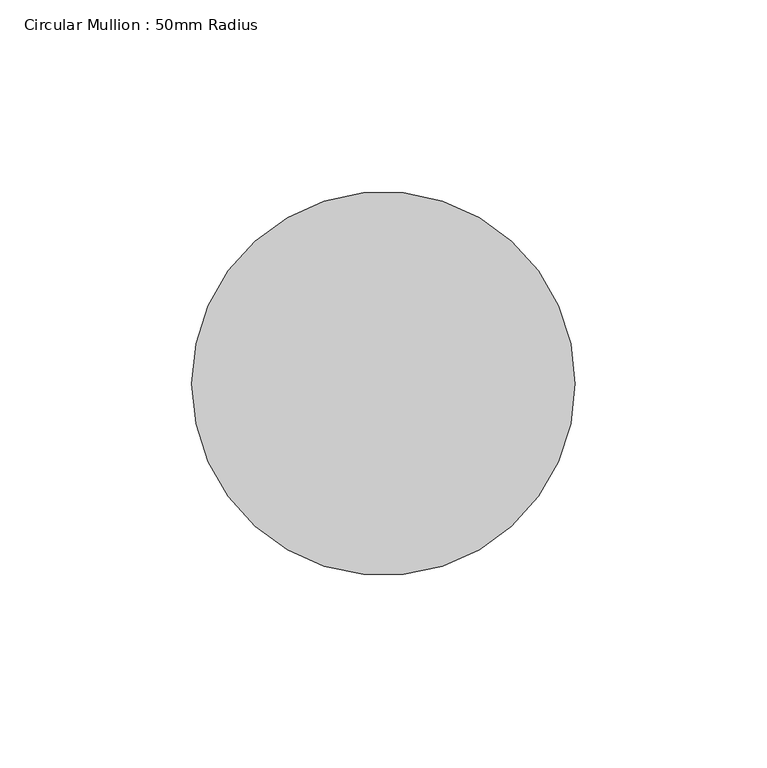
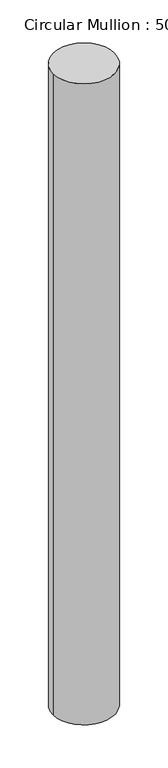
"""IFC4 building model written with IfcOpenShell, lengths in millimetres: member geometry, Circular Mullion : 50mm Radius."""

from ifc_helpers import new_model, si_unit, point, frame, origin, origin_2d, place, context, project, spatial, circle_curve, trimmed, segment, composite_curve, outline, extrude, source, transform, mapped, element, save


def circular_mullion_50mm_radius_9f14a961(model_context):
    return source(origin(), model_context, "Body", "SweptSolid", [
        extrude(outline(composite_curve([segment(trimmed(circle_curve(origin_2d(), 50.0), [point((50.0, 0.0))], [point((-50.0, 0.0))], False, "CARTESIAN"), True, "CONTINUOUS"), segment(trimmed(circle_curve(origin_2d(), 50.0), [point((-50.0, 0.0))], [point((50.0, 0.0))], False, "CARTESIAN"), True, "CONTINUOUS")], self_intersect=False)), frame((0.0, 0.0, -1100.5244759), z_axis=(0.0, 0.0, 1.0), x_axis=(1.0, 0.0, 0.0)), (0.0, 0.0, 1.0), 1100.5244759),
    ])


if __name__ == "__main__":
    model = new_model("IFC4")
    model_context = context("Model", 3, world=origin())
    ifc_project = project(units=[si_unit("LENGTHUNIT", "METRE", prefix="MILLI")], contexts=[model_context])
    site = spatial("IfcSite", under=ifc_project)
    building = spatial("IfcBuilding", under=site)
    placement = place(None, origin())
    circular_mullion_50mm_radius_shape = circular_mullion_50mm_radius_9f14a961(model_context)
    element("IfcMember", 1, ObjectType="Circular Mullion : 50mm Radius", at=placement, inside=building, context=model_context, shape_type="MappedRepresentation", body=[
        mapped(circular_mullion_50mm_radius_shape, transform((0.0, 0.0, 0.0), x_axis=(1.0, 0.0, 0.0), y_axis=(0.0, 1.0, 0.0), z_axis=(0.0, 0.0, 1.0))),
    ])
    save(model, "model.ifc")

# Revit data of these elements
# Type "Circular Mullion : 50mm Radius"
#   built-in parameter 1007350 = 0.164042 (stored number, unit not read)
# Element 1 (IfcMember, "Circular Mullion : 50mm Radius")
#   Materials on its faces: "Aluminium"
# Materials
#   "Aluminium": class "Metal", colour RGB 247 247 247, transparency 0, Description = "Aluminium 6061", Cost = 0
